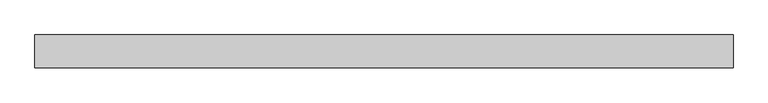
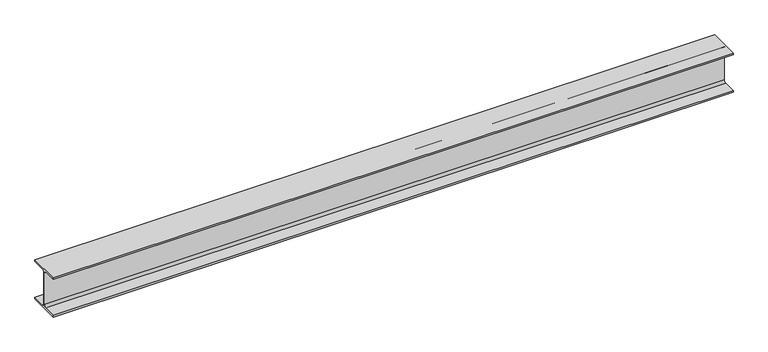
"""IFC4 building model written with IfcOpenShell, lengths in millimetres: beam geometry, 0912_Steel Framing_H-KSD3502 : H_SB_ASB_H-390x300x10x16."""

from ifc_helpers import new_model, si_unit, point, frame, frame_2d, origin, place, context, project, spatial, polyline, circle_curve, trimmed, segment, composite_curve, outline, extrude, source, transform, mapped, element, save


def beam_2561546b(model_context):
    return source(origin(), model_context, "Body", "SweptSolid", [
        extrude(outline(composite_curve([segment(polyline([(150.0, -179.0), (150.0, -195.0), (-150.0, -195.0), (-150.0, -179.0), (-27.0, -179.0)]), True, "CONTINUOUS"), segment(trimmed(circle_curve(frame_2d((-27.0, -157.0)), 22.0), [point((-27.0, -179.0))], [point((-5.0, -157.0))], True, "CARTESIAN"), True, "CONTINUOUS"), segment(polyline([(-5.0, -157.0), (-5.0, 157.0)]), True, "CONTINUOUS"), segment(trimmed(circle_curve(frame_2d((-27.0, 157.0)), 22.0), [point((-5.0, 157.0))], [point((-27.0, 179.0))], True, "CARTESIAN"), True, "CONTINUOUS"), segment(polyline([(-27.0, 179.0), (-150.0, 179.0), (-150.0, 195.0), (150.0, 195.0), (150.0, 179.0), (27.0, 179.0)]), True, "CONTINUOUS"), segment(trimmed(circle_curve(frame_2d((27.0, 157.0)), 22.0), [point((27.0, 179.0))], [point((5.0, 157.0))], True, "CARTESIAN"), True, "CONTINUOUS"), segment(polyline([(5.0, 157.0), (5.0, -157.0)]), True, "CONTINUOUS"), segment(trimmed(circle_curve(frame_2d((27.0, -157.0)), 22.0), [point((5.0, -157.0))], [point((27.0, -179.0))], True, "CARTESIAN"), True, "CONTINUOUS"), segment(polyline([(27.0, -179.0), (150.0, -179.0)]), True, "CONTINUOUS")], self_intersect=False)), frame((-3237.2999994, 0.0, 0.0), z_axis=(1.0, 0.0, 0.0), x_axis=(0.0, 1.0, 0.0)), (0.0, 0.0, 1.0), 6392.0999994),
    ])


if __name__ == "__main__":
    model = new_model("IFC4")
    model_context = context("Model", 3, world=origin())
    ifc_project = project(units=[si_unit("LENGTHUNIT", "METRE", prefix="MILLI")], contexts=[model_context])
    site = spatial("IfcSite", under=ifc_project)
    building = spatial("IfcBuilding", under=site)
    placement = place(None, origin())
    beam_shape = beam_2561546b(model_context)
    element("IfcBeam", 1, ObjectType="0912_Steel Framing_H-KSD3502 : H_SB_ASB_H-390x300x10x16", at=placement, inside=building, context=model_context, shape_type="MappedRepresentation", body=[
        mapped(beam_shape, transform((0.0, 0.0, 0.0), x_axis=(1.0, 0.0, 0.0), y_axis=(0.0, 1.0, 0.0), z_axis=(0.0, 0.0, 1.0))),
    ])
    save(model, "model.ifc")

# Revit data of these elements
# Type "0912_Steel Framing_H-KSD3502 : H_SB_ASB_H-390x300x10x16"
#   H_WM Code_1 = "S01AA001-00001 | Main Steel Structure Fabrication Work | Shelter/Building | Heavy Steel - Standard (Weight≥90KG/M) | Material: (   )"
#   H_WM Code_2 = "S03AA027-00001 | Main Steel Structure Erection Work | Shelter/Building | Heavy Steel (Weight≥90KG/M) | Material: (   )"
#   H_WM Code_3 = "S01AA010-00001 | Main Steel Structure Fabrication Work | Shelter/Building | Steel Painting/Coating | for Non-Fireproofed Steel Surface, Surface Preparation, Primer, Second & Final Coat | Material: (   )"
#   H_Q'ty Cal Type Tag = "SB-Q2"
#   Width = 30.0 cm
#   Web Thickness = 1.0 cm
#   Web Fillet = 2.2 cm
#   Warping Constant = 2520000.0 cm⁶
#   W = 0
#   Torsional Moment of Inertia = 94.3867 cm⁴
#   Section Area = 136.0 cm²
#   Plastic Modulus weak axis = 733.0 cm³
#   Plastic Modulus strong axis = 2190.0 cm³
#   Perimeter = 1.92 m²/m
#   Nominal Weight = 107.00 kgf/m
#   Moment of Inertia weak axis = 7210.00 cm⁴
#   Moment of Inertia strong axis = 38700.00 cm⁴
#   Height = 39.0 cm
#   Flange Thickness = 1.6 cm
#   Elastic Modulus weak axis = 481.0 cm³
#   Elastic Modulus strong axis = 1980.0 cm³
#   Centroid Vertical = 19.5 cm
#   Centroid Horizontal = 15.0 cm
#   Ix = 387000000
#   Length [instance default] = 1.5240 m
#   Zx = 2190000
#   b = 0.3000 m
#   h = 0.3900 m
#   r = 0.0220 m
#   s = 0.0100 m
#   t = 0.0160 m
#   A = 0.0136 m²
#   Structural Material [instance default] = Steel, 45-345
#   Assembly Code = ""
# Element 1 (IfcBeam, "0912_Steel Framing_H-KSD3502 : H_SB_ASB_H-390x300x10x16")
#   Structural Material = none
# Materials
#   "Steel, 45-345": class "Metal", colour RGB 189 187 185, transparency 0, Description = "Steel 345 MPa", Cost = 0
